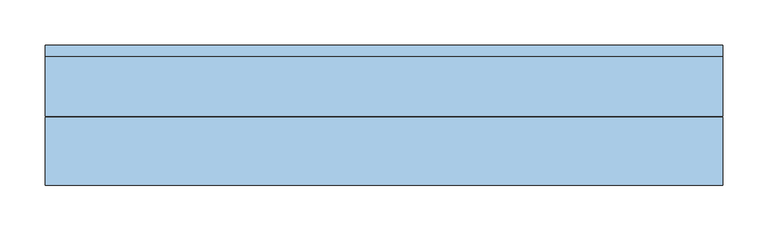
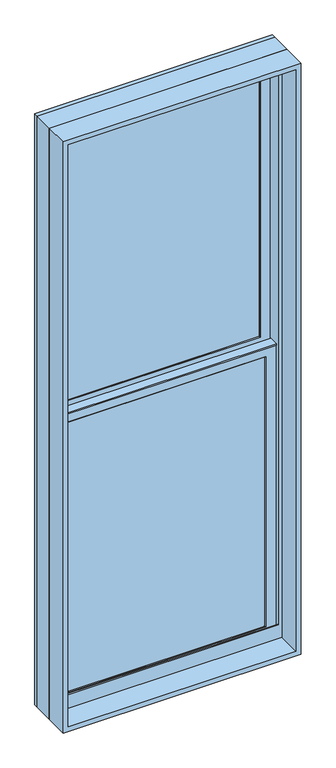
"""IFC4 building model written with IfcOpenShell, lengths in millimetres: window geometry, Window-Double_Hung-Marvin-Essential : ESDH2666."""

import ifcopenshell
import ifcopenshell.guid

model = None  # the IFC model being written
_history = None  # IfcOwnerHistory: only IFC2X3 demands one
_inside = {}  # id of a spatial element -> (the spatial element, [elements in it])
_under = {}  # id of a project, library or spatial element -> (it, [spatial elements below it])
_declared = {}  # id of a project -> (the project, [libraries it declares])
_typed = {}  # id of a type object -> (the type object, [elements of that type])
_made_of = {}  # id of a material, layer set ... -> (it, [elements and type objects made of it])


def new_model(schema):
    """Start an empty IFC model of exactly this schema.

    Asked for "IFC4X3", IfcOpenShell would pick the latest addendum, in which some entities
    have other attributes; the version numbers below select the first issue.
    IFC2X3 requires an IfcOwnerHistory on every rooted entity: one is made here for all.
    """
    global model, _history
    if schema == "IFC4X3":
        model = ifcopenshell.file(schema_version=(4, 3, 0, 0))
    else:
        model = ifcopenshell.file(schema=schema)
    _inside.clear()
    _under.clear()
    _declared.clear()
    _typed.clear()
    _made_of.clear()
    _history = None
    if model.schema == "IFC2X3":
        org = make("IfcOrganization", Name="unknown")
        user = make(
            "IfcPersonAndOrganization",
            ThePerson=make("IfcPerson", FamilyName="unknown"),
            TheOrganization=org,
        )
        app = make(
            "IfcApplication",
            ApplicationDeveloper=org,
            Version="unknown",
            ApplicationFullName="unknown",
            ApplicationIdentifier="unknown",
        )
        _history = make(
            "IfcOwnerHistory",
            OwningUser=user,
            OwningApplication=app,
            ChangeAction="ADDED",
            CreationDate=0,
        )
    return model


def make(cls, **values):
    """One entity of the class cls with the attributes given. An attribute that is None is left unset."""
    return model.create_entity(
        cls, **{name: value for name, value in values.items() if value is not None}
    )


def rooted(cls, **values):
    """An entity with a GlobalId (a new one), such as an element, a storey or a relation."""
    return make(cls, GlobalId=ifcopenshell.guid.new(), OwnerHistory=_history, **values)


def si_unit(unit_type, name, prefix=None):
    """IfcSIUnit, for example si_unit("LENGTHUNIT", "METRE", prefix="MILLI")."""
    return make("IfcSIUnit", UnitType=unit_type, Prefix=prefix, Name=name)


def assignment(units):
    """IfcUnitAssignment: the units of a project."""
    return None if units is None else make("IfcUnitAssignment", Units=units)


def point(xyz):
    """IfcCartesianPoint."""
    return None if xyz is None else make("IfcCartesianPoint", Coordinates=xyz)


def direction(xyz):
    """IfcDirection."""
    return None if xyz is None else make("IfcDirection", DirectionRatios=xyz)


def frame(location, z_axis=None, x_axis=None):
    """IfcAxis2Placement3D, a coordinate frame: its origin and axes. An axis left out is left unset."""
    return make(
        "IfcAxis2Placement3D",
        Location=point(location),
        Axis=direction(z_axis),
        RefDirection=direction(x_axis),
    )


def origin():
    """The frame at (0, 0, 0) with its axes left unset."""
    return frame((0.0, 0.0, 0.0))


def place(relative_to, where):
    """IfcLocalPlacement: puts the frame where relative to a parent placement (None: the world)."""
    return make(
        "IfcLocalPlacement", PlacementRelTo=relative_to, RelativePlacement=where
    )


def context(
    kind, dimensions, precision=None, world=None, true_north=None, identifier=None
):
    """IfcGeometricRepresentationContext, for example the 3D "Model" context."""
    return make(
        "IfcGeometricRepresentationContext",
        ContextIdentifier=identifier,
        ContextType=kind,
        CoordinateSpaceDimension=dimensions,
        Precision=precision,
        WorldCoordinateSystem=world,
        TrueNorth=true_north,
    )


def project(units=None, contexts=None):
    """IfcProject with its units and contexts."""
    return rooted(
        "IfcProject",
        Name="project",
        RepresentationContexts=contexts,
        UnitsInContext=assignment(units),
    )


def spatial(cls, under=None, at=None, **own):
    """A site, building, storey or space (cls), placed at a placement, below another one or the project."""
    s = rooted(cls, ObjectPlacement=at, **own)
    if under is not None:
        _under.setdefault(under.id(), (under, []))[1].append(s)
    return s


def polyline(points):
    """IfcPolyline through the points."""
    return make("IfcPolyline", Points=[point(p) for p in points])


def outline(outer, holes=None, kind="AREA"):
    """IfcArbitraryClosedProfileDef: a profile drawn as a closed curve; with holes, ...WithVoids."""
    if holes is None:
        return make("IfcArbitraryClosedProfileDef", ProfileType=kind, OuterCurve=outer)
    return make(
        "IfcArbitraryProfileDefWithVoids",
        ProfileType=kind,
        OuterCurve=outer,
        InnerCurves=holes,
    )


def extrude(swept, where, along, depth):
    """IfcExtrudedAreaSolid: the profile swept, set in the frame where, extruded along a direction by depth."""
    return make(
        "IfcExtrudedAreaSolid",
        SweptArea=swept,
        Position=where,
        ExtrudedDirection=direction(along),
        Depth=depth,
    )


def faces_of(points, faces, orient=None, outer=None):
    """IfcFace entities. A face is a list of loops; a loop is a list of indices into points, from 0.

    orient and outer hold one flag for each loop. By default every Orientation is true, the
    first loop of a face is its IfcFaceOuterBound and the others are IfcFaceBound.
    """
    made = []
    for i, loops in enumerate(faces):
        bounds = []
        for j, loop in enumerate(loops):
            is_outer = j == 0 if outer is None else outer[i][j]
            bounds.append(
                make(
                    "IfcFaceOuterBound" if is_outer else "IfcFaceBound",
                    Bound=make("IfcPolyLoop", Polygon=[points[k] for k in loop]),
                    Orientation=True if orient is None else orient[i][j],
                )
            )
        made.append(make("IfcFace", Bounds=bounds))
    return made


def faceted_brep(points, faces, orient=None, outer=None, voids=None):
    """IfcFacetedBrep: a solid bounded by flat faces; with voids (closed shells), ...WithVoids."""
    shared = [point(p) for p in points]
    hull = make("IfcClosedShell", CfsFaces=faces_of(shared, faces, orient, outer))
    if voids is None:
        return make("IfcFacetedBrep", Outer=hull)
    return make(
        "IfcFacetedBrepWithVoids",
        Outer=hull,
        Voids=[
            make(cls, CfsFaces=faces_of(shared, fs, o, b)) for cls, fs, o, b in voids
        ],
    )


def shape(context_of_items, identifier, shape_type, items):
    """IfcShapeRepresentation: the items that make up one representation, for example the "Body"."""
    return make(
        "IfcShapeRepresentation",
        ContextOfItems=context_of_items,
        RepresentationIdentifier=identifier,
        RepresentationType=shape_type,
        Items=items,
    )


def source(mapping_origin, context_of_items, identifier, shape_type, items):
    """IfcRepresentationMap: a shape defined once, which mapped items show again and again."""
    return make(
        "IfcRepresentationMap",
        MappingOrigin=mapping_origin,
        MappedRepresentation=shape(context_of_items, identifier, shape_type, items),
    )


def transform(
    local_origin,
    x_axis=None,
    y_axis=None,
    z_axis=None,
    scale=None,
    scale2=None,
    scale3=None,
    uniform=True,
):
    """IfcCartesianTransformationOperator3D, or its non-uniform kind. x_axis, y_axis, z_axis: its Axis1, 2, 3."""
    if uniform:
        return make(
            "IfcCartesianTransformationOperator3D",
            Axis1=direction(x_axis),
            Axis2=direction(y_axis),
            LocalOrigin=point(local_origin),
            Scale=scale,
            Axis3=direction(z_axis),
        )
    return make(
        "IfcCartesianTransformationOperator3DnonUniform",
        Axis1=direction(x_axis),
        Axis2=direction(y_axis),
        LocalOrigin=point(local_origin),
        Scale=scale,
        Axis3=direction(z_axis),
        Scale2=scale2,
        Scale3=scale3,
    )


def mapped(mapping_source, mapping_target):
    """IfcMappedItem: shows the shape of a source again, moved by a transform."""
    return make(
        "IfcMappedItem", MappingSource=mapping_source, MappingTarget=mapping_target
    )


def made_of(thing, what):
    """Note that an element or type object is made of a material, layer set ...; save() writes the relation."""
    if what is not None:
        _made_of.setdefault(what.id(), (what, []))[1].append(thing)
    return thing


def element(
    cls,
    number,
    at=None,
    inside=None,
    cuts=None,
    type_object=None,
    material=None,
    context=None,
    identifier="Body",
    shape_type=None,
    held_by="IfcProductDefinitionShape",
    body=None,
    shapes=None,
    **own,
):
    """One element of the class cls, such as IfcWall. Its Tag is "e" and its number.

    at: its placement. inside: the storey or other place that contains it. cuts: it is an
    opening in that element (IfcRelVoidsElement). A single representation is given by context,
    identifier, shape_type and body (its items); several are given by shapes. held_by: the class
    of the entity that holds the representations. save() writes the other relations.
    """
    e = rooted(cls, Tag="e%d" % number, ObjectPlacement=at, **own)
    if body is not None:
        shapes = [shape(context, identifier, shape_type, body)]
    if shapes is not None:
        e.Representation = make(held_by, Representations=shapes)
    if inside is not None:
        _inside.setdefault(inside.id(), (inside, []))[1].append(e)
    if cuts is not None:
        rooted(
            "IfcRelVoidsElement", RelatingBuildingElement=cuts, RelatedOpeningElement=e
        )
    if type_object is not None:
        _typed.setdefault(type_object.id(), (type_object, []))[1].append(e)
    return made_of(e, material)


def aggregate(whole, parts):
    """IfcRelAggregates: a whole, such as a stair, and the parts it consists of."""
    return rooted("IfcRelAggregates", RelatingObject=whole, RelatedObjects=parts)


def save(model, path):
    """Write the relations noted so far, then the file.

    IfcRelAggregates (storeys below a building ...), IfcRelContainedInSpatialStructure (elements
    in a storey), IfcRelDefinesByType, IfcRelAssociatesMaterial and IfcRelDeclares: one each for
    every whole, place, type object, material and project.
    """
    for whole, parts in _under.values():
        aggregate(whole, parts)
    for where, things in _inside.values():
        rooted(
            "IfcRelContainedInSpatialStructure",
            RelatedElements=things,
            RelatingStructure=where,
        )
    for kind, things in _typed.values():
        rooted("IfcRelDefinesByType", RelatedObjects=things, RelatingType=kind)
    for what, things in _made_of.values():
        rooted("IfcRelAssociatesMaterial", RelatedObjects=things, RelatingMaterial=what)
    for by, libraries in _declared.values():
        rooted("IfcRelDeclares", RelatingContext=by, RelatedDefinitions=libraries)
    model.write(path)


def window_a1344563(model_context):
    return source(origin(), model_context, "Body", "SolidModel", [
        extrude(outline(polyline([(115.3583333, 20.6375), (115.3583333, 15.875), (96.3083333, 15.875), (96.3083333, 20.6375), (115.3583333, 20.6375)])), frame((0.0, 0.0, 527.05), z_axis=(0.0, 0.0, 1.0), x_axis=(1.0, 0.0, 0.0)), (0.0, 0.0, 1.0), 908.05),
        extrude(outline(polyline([(-96.3083333, 20.6375), (-96.3083333, 15.875), (-115.3583333, 15.875), (-115.3583333, 20.6375), (-96.3083333, 20.6375)])), frame((0.0, 0.0, 527.05), z_axis=(0.0, 0.0, 1.0), x_axis=(1.0, 0.0, 0.0)), (0.0, 0.0, 1.0), 908.05),
        extrude(outline(polyline([(317.5, 20.6375), (317.5, 15.875), (-317.5, 15.875), (-317.5, 20.6375), (317.5, 20.6375)])), frame((0.0, 0.0, 971.55), z_axis=(0.0, 0.0, 1.0), x_axis=(1.0, 0.0, 0.0)), (0.0, 0.0, 1.0), 19.05),
        extrude(outline(polyline([(-115.3583333, 46.83125), (-115.3583333, 51.59375), (-96.3083333, 51.59375), (-96.3083333, 46.83125), (-115.3583333, 46.83125)])), frame((0.0, 0.0, 1473.2), z_axis=(0.0, 0.0, 1.0), x_axis=(1.0, 0.0, 0.0)), (0.0, 0.0, 1.0), 908.05),
        extrude(outline(polyline([(96.3083333, 46.83125), (96.3083333, 51.59375), (115.3583333, 51.59375), (115.3583333, 46.83125), (96.3083333, 46.83125)])), frame((0.0, 0.0, 1473.2), z_axis=(0.0, 0.0, 1.0), x_axis=(1.0, 0.0, 0.0)), (0.0, 0.0, 1.0), 908.05),
        extrude(outline(polyline([(-317.5, 46.83125), (-317.5, 51.59375), (317.5, 51.59375), (317.5, 46.83125), (-317.5, 46.83125)])), frame((0.0, 0.0, 1917.7), z_axis=(0.0, 0.0, 1.0), x_axis=(1.0, 0.0, 0.0)), (0.0, 0.0, 1.0), 19.05),
        extrude(outline(polyline([(115.3583333, 20.6375), (96.3083333, 20.6375), (96.3083333, 25.4), (115.3583333, 25.4), (115.3583333, 20.6375)])), frame((0.0, 0.0, 527.05), z_axis=(0.0, 0.0, 1.0), x_axis=(1.0, 0.0, 0.0)), (0.0, 0.0, 1.0), 908.05),
        extrude(outline(polyline([(-96.3083333, 20.6375), (-115.3583333, 20.6375), (-115.3583333, 25.4), (-96.3083333, 25.4), (-96.3083333, 20.6375)])), frame((0.0, 0.0, 527.05), z_axis=(0.0, 0.0, 1.0), x_axis=(1.0, 0.0, 0.0)), (0.0, 0.0, 1.0), 908.05),
        extrude(outline(polyline([(317.5, 20.6375), (-317.5, 20.6375), (-317.5, 25.4), (317.5, 25.4), (317.5, 20.6375)])), frame((0.0, 0.0, 971.55), z_axis=(0.0, 0.0, 1.0), x_axis=(1.0, 0.0, 0.0)), (0.0, 0.0, 1.0), 19.05),
        extrude(outline(polyline([(-115.3583333, 56.35625), (-96.3083333, 56.35625), (-96.3083333, 51.59375), (-115.3583333, 51.59375), (-115.3583333, 56.35625)])), frame((0.0, 0.0, 1473.2), z_axis=(0.0, 0.0, 1.0), x_axis=(1.0, 0.0, 0.0)), (0.0, 0.0, 1.0), 908.05),
        extrude(outline(polyline([(96.3083333, 56.35625), (115.3583333, 56.35625), (115.3583333, 51.59375), (96.3083333, 51.59375), (96.3083333, 56.35625)])), frame((0.0, 0.0, 1473.2), z_axis=(0.0, 0.0, 1.0), x_axis=(1.0, 0.0, 0.0)), (0.0, 0.0, 1.0), 908.05),
        extrude(outline(polyline([(-317.5, 56.35625), (317.5, 56.35625), (317.5, 51.59375), (-317.5, 51.59375), (-317.5, 56.35625)])), frame((0.0, 0.0, 1917.7), z_axis=(0.0, 0.0, 1.0), x_axis=(1.0, 0.0, 0.0)), (0.0, 0.0, 1.0), 19.05),
        faceted_brep([(-344.4875, 5.6780605, 1465.1351748), (-344.4875, 5.6780605, 1460.5), (344.4875, 5.6780605, 1460.5), (344.4875, 5.6780605, 1465.1351748), (-344.4875, 34.8118605, 1465.1351748), (344.4875, 34.8118605, 1465.1351748), (344.4875, 34.8118605, 1460.5), (-344.4875, 34.8118605, 1460.5), (-344.4875, 30.1625, 1460.5), (-344.4875, 30.1625, 500.0625), (-344.4875, 8.9241104, 500.0625), (-344.4875, 8.9241104, 1460.5), (344.4875, 8.9241104, 1460.5), (344.4875, 30.1625, 1460.5), (344.4875, 8.9241104, 500.0625), (344.4875, 30.1625, 500.0625), (-328.6034752, 11.90625, 1446.2034752), (-328.6034752, 30.1625, 1446.2034752), (328.6034752, 30.1625, 1446.2034752), (328.6034752, 11.90625, 1446.2034752), (-311.94375, 10.4662439, 1429.54375), (-311.94375, 11.90625, 1429.54375), (311.94375, 11.90625, 1429.54375), (311.94375, 10.4662439, 1429.54375), (313.4858834, 8.9241104, 1431.0858834), (-313.4858834, 8.9241104, 1431.0858834), (328.6034752, 30.1625, 515.9465248), (328.6034752, 11.90625, 515.9465248), (311.94375, 11.90625, 532.60625), (311.94375, 10.4662439, 532.60625), (313.4858834, 8.9241104, 531.0641166), (-328.6034752, 30.1625, 515.9465248), (-328.6034752, 11.90625, 515.9465248), (-311.94375, 11.90625, 532.60625), (-311.94375, 10.4662439, 532.60625), (-313.4858834, 8.9241104, 531.0641166)], [[[0, 1, 2, 3]], [[4, 5, 6, 7]], [[1, 0, 4, 7, 8, 9, 10, 11]], [[2, 1, 11, 12]], [[7, 6, 13, 8]], [[3, 2, 12, 14, 15, 13, 6, 5]], [[0, 3, 5, 4]], [[16, 17, 18, 19]], [[20, 21, 22, 23]], [[20, 23, 24, 25]], [[19, 18, 26, 27]], [[23, 22, 28, 29]], [[24, 23, 29, 30]], [[27, 26, 31, 32]], [[29, 28, 33, 34]], [[30, 29, 34, 35]], [[15, 14, 10, 9]], [[15, 9, 8, 13], [18, 17, 31, 26]], [[17, 16, 32, 31]], [[16, 19, 27, 32], [22, 21, 33, 28]], [[21, 20, 34, 33]], [[20, 25, 35, 34]], [[10, 14, 12, 11], [25, 24, 30, 35]]]),
        extrude(outline(polyline([(38.5955581, 1446.2125), (33.5778968, 1446.2125), (33.5778968, 1447.8), (39.9405976, 1447.8), (39.9405976, 1446.2125), (61.515625, 1446.2125), (47.6307501, 1442.8975159), (38.5955581, 1442.8975159), (38.5955581, 1446.2125)])), frame((-344.4875, 0.0, 0.0), z_axis=(1.0, 0.0, 0.0), x_axis=(0.0, 1.0, 0.0)), (0.0, 0.0, 1.0), 688.975),
        faceted_brep([(374.65, 0.0, 469.9), (374.65, 0.0, 2438.4), (-374.65, 0.0, 2438.4), (-374.65, 0.0, 469.9), (348.45625, 0.0, 531.01875), (-348.45625, 0.0, 531.01875), (-348.45625, 0.0, 2412.20625), (348.45625, 0.0, 2412.20625), (348.45625, 3.96875, 469.9), (-348.45625, 3.96875, 469.9), (-348.45625, 3.96875, 531.01875), (348.45625, 3.96875, 531.01875), (-374.65, 65.6828125, 469.9), (-348.45625, 65.6828125, 469.9), (348.45625, 65.6828125, 469.9), (374.65, 65.6828125, 469.9), (-374.65, 65.6828125, 2438.4), (374.65, 65.6828125, 2438.4), (348.45625, 65.6828125, 2412.20625), (-348.45625, 65.6828125, 2412.20625)], [[[0, 1, 2, 3], [4, 5, 6, 7]], [[8, 9, 10, 11]], [[5, 4, 11, 10]], [[0, 3, 12, 13, 9, 8, 14, 15]], [[13, 12, 16, 17, 15, 14, 18, 19]], [[13, 19, 6, 5, 10, 9]], [[7, 6, 19, 18]], [[18, 14, 8, 11, 4, 7]], [[1, 0, 15, 17]], [[2, 1, 17, 16]], [[3, 2, 16, 12]]]),
        faceted_brep([(348.45625, 30.1625, 1454.15), (346.86875, 30.1625, 1454.15), (346.86875, 30.1625, 494.2544613), (348.45625, 30.1625, 494.2544613), (-346.86875, 30.1625, 1454.15), (-348.45625, 30.1625, 1454.15), (-348.45625, 30.1625, 494.2544613), (-346.86875, 30.1625, 494.2544613), (346.86875, 63.5, 1454.15), (348.45625, 63.5, 1454.15), (348.45625, 63.5, 487.7743077), (346.86875, 63.5, 487.7743077), (-348.45625, 63.5, 1454.15), (-346.86875, 63.5, 1454.15), (-346.86875, 63.5, 487.7743077), (-348.45625, 63.5, 487.7743077), (359.7108932, 3.96875, 499.3460105), (359.7108932, 3.96875, 469.9), (359.7108932, 65.6828125, 469.9), (359.7108932, 65.6828125, 487.350012), (-359.7108932, 3.96875, 469.9), (-359.7108932, 3.96875, 499.3460105), (-359.7108932, 65.6828125, 487.350012), (-359.7108932, 65.6828125, 469.9), (359.7108932, 78.58125, 484.8428097), (-359.7108932, 78.58125, 484.8428097), (-357.6971252, 68.2348864, 486.8539391), (-339.73135, 68.2348864, 486.8539391), (-339.73135, 65.6828125, 487.350012), (339.73135, 65.6828125, 487.350012), (339.73135, 68.2348864, 486.8539391), (357.6971252, 68.2348864, 486.8539391), (-374.65, 65.6828125, 469.9), (-374.65, 78.5948249, 469.9), (374.65, 78.5948249, 469.9), (374.65, 65.6828125, 469.9), (-374.65, 78.58125, 2438.4), (374.65, 78.58125, 2438.4), (359.7108932, 78.58125, 2423.4608932), (-359.7108932, 78.58125, 2423.4608932), (-374.65, 65.6828125, 2438.4), (-357.6971252, 68.2348864, 2421.4471252), (357.6971252, 68.2348864, 2421.4471252), (339.73135, 68.2348864, 2403.48135), (-339.73135, 68.2348864, 2403.48135), (-339.73135, 65.6828125, 2403.48135), (339.73135, 65.6828125, 2403.48135), (374.65, 65.6828125, 2438.4)], [[[0, 1, 2, 3]], [[4, 5, 6, 7]], [[8, 9, 10, 11]], [[12, 13, 14, 15]], [[1, 8, 11, 2]], [[9, 0, 3, 10]], [[1, 0, 9, 8]], [[5, 4, 13, 12]], [[5, 12, 15, 6]], [[13, 4, 7, 14]], [[16, 17, 18, 19]], [[20, 21, 22, 23]], [[24, 25, 26, 27, 28, 22, 21, 16, 19, 29, 30, 31], [3, 2, 11, 10], [7, 6, 15, 14]], [[17, 16, 21, 20]], [[17, 20, 23, 32, 33, 34, 35, 18]], [[34, 33, 36, 37], [25, 24, 38, 39]], [[33, 32, 40, 36]], [[39, 41, 26, 25]], [[41, 42, 31, 30, 43, 44, 27, 26]], [[44, 45, 28, 27]], [[40, 32, 23, 22, 28, 45, 46, 29, 19, 18, 35, 47]], [[36, 40, 47, 37]], [[39, 38, 42, 41]], [[44, 43, 46, 45]], [[34, 37, 47, 35]], [[42, 38, 24, 31]], [[46, 43, 30, 29]]]),
        extrude(outline(polyline([(324.64375, 11.90625), (-324.64375, 11.90625), (-324.64375, 15.08125), (324.64375, 15.08125), (324.64375, 11.90625)])), frame((0.0, 0.0, 519.90625), z_axis=(0.0, 0.0, 1.0), x_axis=(1.0, 0.0, 0.0)), (0.0, 0.0, 1.0), 922.3375),
        extrude(outline(polyline([(324.64375, 42.8625), (-324.64375, 42.8625), (-324.64375, 46.0375), (324.64375, 46.0375), (324.64375, 42.8625)])), frame((0.0, 0.0, 1466.05625), z_axis=(0.0, 0.0, 1.0), x_axis=(1.0, 0.0, 0.0)), (0.0, 0.0, 1.0), 922.3375),
        faceted_brep([(-311.94375, 31.194477, 1429.54375), (-313.4858834, 32.7366104, 1431.0858834), (313.4858834, 32.7366104, 1431.0858834), (311.94375, 31.194477, 1429.54375), (-311.94375, 30.1625, 1429.54375), (311.94375, 30.1625, 1429.54375), (-344.4875, 32.7366104, 1462.0875), (-344.4875, 30.1625, 1462.0875), (344.4875, 30.1625, 1462.0875), (344.4875, 32.7366104, 1462.0875), (313.4858834, 32.7366104, 531.0641166), (311.94375, 31.194477, 532.60625), (311.94375, 30.1625, 532.60625), (344.4875, 30.1625, 500.0625), (344.4875, 32.7366104, 500.0625), (-313.4858834, 32.7366104, 531.0641166), (-311.94375, 31.194477, 532.60625), (-311.94375, 30.1625, 532.60625), (-344.4875, 30.1625, 500.0625), (-344.4875, 32.7366104, 500.0625)], [[[0, 1, 2, 3]], [[4, 0, 3, 5]], [[6, 7, 8, 9]], [[3, 2, 10, 11]], [[5, 3, 11, 12]], [[9, 8, 13, 14]], [[11, 10, 15, 16]], [[12, 11, 16, 17]], [[14, 13, 18, 19]], [[9, 14, 19, 6], [1, 15, 10, 2]], [[16, 15, 1, 0]], [[17, 16, 0, 4]], [[7, 18, 13, 8], [5, 12, 17, 4]], [[19, 18, 7, 6]]]),
        faceted_brep([(-328.6034752, 42.8625, 2392.3534752), (-328.6034752, 61.11875, 2392.3534752), (328.6034752, 61.11875, 2392.3534752), (328.6034752, 42.8625, 2392.3534752), (-311.94375, 41.4224939, 2375.69375), (-311.94375, 42.8625, 2375.69375), (311.94375, 42.8625, 2375.69375), (311.94375, 41.4224939, 2375.69375), (-313.4858834, 39.8803604, 2377.2358834), (313.4858834, 39.8803604, 2377.2358834), (-344.4875, 61.11875, 2408.2375), (-344.4875, 39.8803604, 2408.2375), (344.4875, 39.8803604, 2408.2375), (344.4875, 61.11875, 2408.2375), (328.6034752, 61.11875, 1462.0965248), (328.6034752, 42.8625, 1462.0965248), (311.94375, 42.8625, 1478.75625), (311.94375, 41.4224939, 1478.75625), (313.4858834, 39.8803604, 1477.2141166), (344.4875, 39.8803604, 1446.2125), (344.4875, 61.11875, 1446.2125), (-328.6034752, 61.11875, 1462.0965248), (-328.6034752, 42.8625, 1462.0965248), (-311.94375, 42.8625, 1478.75625), (-311.94375, 41.4224939, 1478.75625), (-313.4858834, 39.8803604, 1477.2141166), (-344.4875, 39.8803604, 1446.2125), (-344.4875, 61.11875, 1446.2125)], [[[0, 1, 2, 3]], [[4, 5, 6, 7]], [[8, 4, 7, 9]], [[10, 11, 12, 13]], [[3, 2, 14, 15]], [[7, 6, 16, 17]], [[9, 7, 17, 18]], [[13, 12, 19, 20]], [[15, 14, 21, 22]], [[17, 16, 23, 24]], [[18, 17, 24, 25]], [[20, 19, 26, 27]], [[13, 20, 27, 10], [1, 21, 14, 2]], [[22, 21, 1, 0]], [[3, 15, 22, 0], [5, 23, 16, 6]], [[24, 23, 5, 4]], [[25, 24, 4, 8]], [[11, 26, 19, 12], [9, 18, 25, 8]], [[27, 26, 11, 10]]]),
        faceted_brep([(-344.4875, 61.11875, 1446.2125), (-344.4875, 63.6928604, 1446.2125), (344.4875, 63.6928604, 1446.2125), (344.4875, 61.11875, 1446.2125), (-311.94375, 62.150727, 1478.75625), (-311.94375, 61.11875, 1478.75625), (311.94375, 61.11875, 1478.75625), (311.94375, 62.150727, 1478.75625), (-313.4858834, 63.6928604, 1477.2141166), (313.4858834, 63.6928604, 1477.2141166), (344.4875, 63.6928604, 2408.2375), (344.4875, 61.11875, 2408.2375), (311.94375, 61.11875, 2375.69375), (311.94375, 62.150727, 2375.69375), (313.4858834, 63.6928604, 2377.2358834), (-344.4875, 63.6928604, 2408.2375), (-344.4875, 61.11875, 2408.2375), (-311.94375, 61.11875, 2375.69375), (-311.94375, 62.150727, 2375.69375), (-313.4858834, 63.6928604, 2377.2358834)], [[[0, 1, 2, 3]], [[4, 5, 6, 7]], [[8, 4, 7, 9]], [[3, 2, 10, 11]], [[7, 6, 12, 13]], [[9, 7, 13, 14]], [[11, 10, 15, 16]], [[13, 12, 17, 18]], [[14, 13, 18, 19]], [[16, 15, 1, 0]], [[3, 11, 16, 0], [5, 17, 12, 6]], [[18, 17, 5, 4]], [[19, 18, 4, 8]], [[1, 15, 10, 2], [9, 14, 19, 8]]]),
        extrude(outline(polyline([(324.64375, 26.19375), (-324.64375, 26.19375), (-324.64375, 30.1625), (324.64375, 30.1625), (324.64375, 26.19375)])), frame((0.0, 0.0, 519.90625), z_axis=(0.0, 0.0, 1.0), x_axis=(1.0, 0.0, 0.0)), (0.0, 0.0, 1.0), 922.3375),
        extrude(outline(polyline([(324.64375, 57.15), (-324.64375, 57.15), (-324.64375, 61.11875), (324.64375, 61.11875), (324.64375, 57.15)])), frame((0.0, 0.0, 1466.05625), z_axis=(0.0, 0.0, 1.0), x_axis=(1.0, 0.0, 0.0)), (0.0, 0.0, 1.0), 922.3375),
        extrude(outline(polyline([(2438.4, 374.65), (2438.4, -374.65), (469.9, -374.65), (469.9, 374.65), (2438.4, 374.65)]), holes=[polyline([(2422.525, 358.775), (485.775, 358.775), (485.775, -358.775), (2422.525, -358.775), (2422.525, 358.775)])]), frame((0.0, -76.2, 0.0), z_axis=(0.0, 1.0, 0.0), x_axis=(0.0, 0.0, 1.0)), (0.0, 0.0, 1.0), 75.40625),
    ])


if __name__ == "__main__":
    model = new_model("IFC4")
    model_context = context("Model", 3, world=origin())
    ifc_project = project(units=[si_unit("LENGTHUNIT", "METRE", prefix="MILLI")], contexts=[model_context])
    site = spatial("IfcSite", under=ifc_project)
    building = spatial("IfcBuilding", under=site)
    placement = place(None, origin())
    window_shape = window_a1344563(model_context)
    element("IfcWindow", 1, ObjectType="Window-Double_Hung-Marvin-Essential : ESDH2666", at=placement, inside=building, context=model_context, shape_type="MappedRepresentation", body=[
        mapped(window_shape, transform((0.0, 0.0, 0.0), x_axis=(1.0, 0.0, 0.0), y_axis=(0.0, 1.0, 0.0), z_axis=(0.0, 0.0, 1.0))),
    ])
    save(model, "model.ifc")

# Revit data of these elements
# Type "Window-Double_Hung-Marvin-Essential : ESDH2666"
#   Type Mark = "84"
#   Window Type = "Essential Double Hung"
#   Product data url = "https://bimobject.com/marvin-windows-and-doors/product/marvin-dhwau"
#   Product Guid = "c4a96547-874c-4385-91dc-a058adc19d98"
#   Frame = "All Ultrex"
#   Egress Window = "Yes"
#   URL = "www.marvin.com"
#   Model = "ESDH2666"
#   Manufacturer = "Marvin Windows and Doors"
#   Label Egress = "EGRESS WDW"
#   Glass Type = "IG Low E II with Argon"
#   Design Pressure = "DP40"
#   Description = "3078 DBHG"
#   Analytic Construction = "<None>"
#   Prairie Corner Width = 0' - 4"
#   Prairie Corner Height = 0' - 4"
#   Egress Width = 2' - 2 9/16"
#   Egress Height = 2' - 10 27/128"
#   Rough Width = 2' - 6"
#   Rough Height = 6' - 6"
#   Nominal Width = 2' - 6"
#   Nominal Height = 6' - 6"
#   Inset to Installation Flange [instance default] = 0' - 1"
#   Height = 6' - 5 1/2"
#   Egress Area = 6.31061 SF
#   Default Head Height = 8' - 0"
#   Width = 2' - 5 1/2"
#   Daylight Area = 12.0467 SF
#   DLO Width = 2' - 0 9/16"
#   DLO Height = 2' - 11 5/16"
#   Muntins Top Sash = yes
#   Lites Wide Top Sash = 3
#   Lites Wide Bottom Sash = 3
#   Lites High Top Sash = 2
#   Lites High Bottom Sash = 2
#   Lite Cut Prairie 9 = no
#   Lite Cut HV Grid = yes
#   Muntins Bottom Sash = yes
#   Label Visibility = no
#   Jamb Extension Visibility = yes
#   Edition number = 1
#   Interior Material = Ultrex-Marvin-Stonewhite
#   Glazing Material = Glass-Marvin-IG Low E II with Argon
#   Cladding Material = Ultrex-Marvin-Pebblegray
#   Wall Closure = (empty or 0)
#   Assembly Code = ""
# Element 1 (IfcWindow, "Window-Double_Hung-Marvin-Essential : ESDH2666")
#   Materials on its faces: "Ultrex-Marvin-Pebblegray", "Ultrex-Marvin-Stonewhite", "Glass-Marvin-IG Low E II with Argon"
# Materials
#   "Ultrex-Marvin-Stonewhite": class "Paint", colour RGB 250 251 245, transparency 0
#   "Glass-Marvin-IG Low E II with Argon": class "Glass", colour RGB 0 128 192, transparency 0.85
#   "Ultrex-Marvin-Pebblegray": class "Paint", colour RGB 189 185 173, transparency 0
